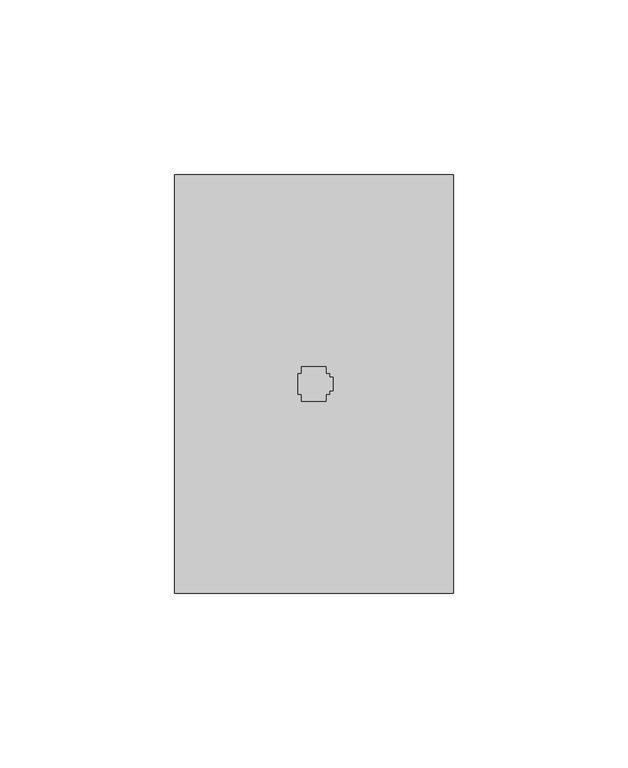
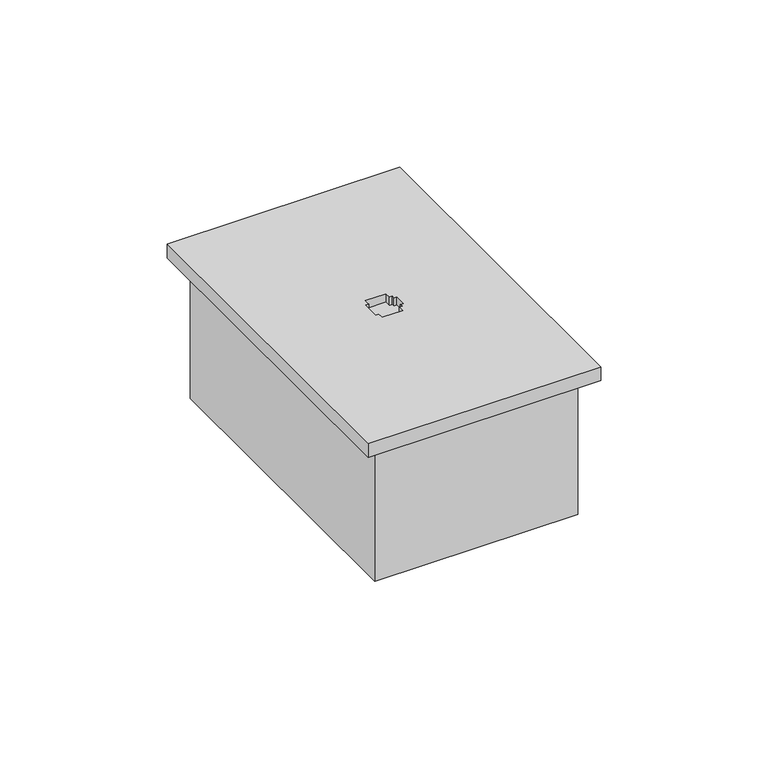
"""IFC4 building model written with IfcOpenShell, lengths in millimetres: proxy geometry, CAIXA VERTICE V7 : Telefone."""

from ifc_helpers import new_model, si_unit, origin, place, context, project, spatial, faceted_brep, source, transform, mapped, element, save


def electrical_fixtures_d1a6b59b(model_context):
    return source(origin(), model_context, "Body", "Brep", [
        faceted_brep([(33.0, 247.0, -48.0), (33.0, 353.0, -48.0), (-33.0, 353.0, -48.0), (-33.0, 247.0, -48.0), (35.0, 355.0, -50.0), (35.0, 245.0, -50.0), (-35.0, 245.0, -50.0), (-35.0, 355.0, -50.0), (-35.0, 355.0, 0.0), (35.0, 355.0, 0.0), (-35.0, 245.0, 0.0), (35.0, 245.0, 0.0), (33.0, 353.0, 0.0), (33.0, 247.0, 0.0), (-33.0, 247.0, 0.0), (-33.0, 353.0, 0.0)], [[[0, 1, 2, 3]], [[4, 5, 6, 7]], [[4, 7, 8, 9]], [[8, 7, 6, 10]], [[10, 6, 5, 11]], [[11, 5, 4, 9]], [[9, 8, 10, 11], [12, 13, 14, 15]], [[13, 12, 1, 0]], [[14, 13, 0, 3]], [[15, 14, 3, 2]], [[12, 15, 2, 1]]]),
        faceted_brep([(40.0, 360.0, 5.0), (-40.0, 360.0, 5.0), (-40.0, 240.0, 5.0), (40.0, 240.0, 5.0), (-3.5, 303.0, 5.0), (-3.5, 305.0, 5.0), (3.5, 305.0, 5.0), (3.5, 303.0, 5.0), (4.5, 303.0, 5.0), (4.5, 302.0, 5.0), (5.5, 302.0, 5.0), (5.5, 298.0, 5.0), (4.5, 298.0, 5.0), (4.5, 297.0, 5.0), (3.5, 297.0, 5.0), (3.5, 295.0, 5.0), (-3.5, 295.0, 5.0), (-3.5, 297.0, 5.0), (-4.5, 297.0, 5.0), (-4.5, 303.0, 5.0), (-40.0, 360.0, 0.0), (40.0, 360.0, 0.0), (40.0, 240.0, 0.0), (-40.0, 240.0, 0.0), (-3.5, 303.0, 2.0), (-3.5, 305.0, 2.0), (-4.5, 303.0, 2.0), (-4.5, 297.0, 2.0), (-3.5, 297.0, 2.0), (-3.5, 295.0, 2.0), (3.5, 295.0, 2.0), (3.5, 297.0, 2.0), (3.5, 305.0, 2.0), (4.5, 297.0, 2.0), (4.5, 298.0, 2.0), (5.5, 298.0, 2.0), (5.5, 302.0, 2.0), (4.5, 302.0, 2.0), (4.5, 303.0, 2.0), (3.5, 303.0, 2.0)], [[[0, 1, 2, 3], [4, 5, 6, 7, 8, 9, 10, 11, 12, 13, 14, 15, 16, 17, 18, 19]], [[20, 21, 22, 23]], [[1, 0, 21, 20]], [[2, 1, 20, 23]], [[3, 2, 23, 22]], [[0, 3, 22, 21]], [[24, 25, 5, 4]], [[26, 24, 4, 19]], [[27, 26, 19, 18]], [[28, 27, 18, 17]], [[29, 28, 17, 16]], [[30, 29, 16, 15]], [[31, 30, 15, 14]], [[32, 25, 24, 26, 27, 28, 29, 30, 31, 33, 34, 35, 36, 37, 38, 39]], [[25, 32, 6, 5]], [[33, 31, 14, 13]], [[34, 33, 13, 12]], [[35, 34, 12, 11]], [[36, 35, 11, 10]], [[37, 36, 10, 9]], [[38, 37, 9, 8]], [[39, 38, 8, 7]], [[32, 39, 7, 6]]]),
    ])


if __name__ == "__main__":
    model = new_model("IFC4")
    model_context = context("Model", 3, world=origin())
    ifc_project = project(units=[si_unit("LENGTHUNIT", "METRE", prefix="MILLI")], contexts=[model_context])
    site = spatial("IfcSite", under=ifc_project)
    building = spatial("IfcBuilding", under=site)
    placement = place(None, origin())
    electrical_fixtures_shape = electrical_fixtures_d1a6b59b(model_context)
    element("IfcBuildingElementProxy", 1, Name="CAIXA VERTICE V7 : Telefone", ObjectType="CAIXA VERTICE V7 : Telefone", at=placement, inside=building, context=model_context, shape_type="MappedRepresentation", body=[
        mapped(electrical_fixtures_shape, transform((0.0, 0.0, 0.0), x_axis=(1.0, 0.0, 0.0), y_axis=(0.0, 1.0, 0.0), z_axis=(0.0, 0.0, 1.0))),
    ])
    save(model, "model.ifc")

# Revit data of these elements
# Type "CAIXA VERTICE V7 : Telefone"
#   URL = "www.facebook.com/verticetreinamentos"
#   SEÇÃO [instance default] = ""
#   Rotação [instance default] = 0.00°
#   LARGURA DA TAMPA = 0.08 m
#   BORDA = 0.01 m
#   ALTURA DE INSTALAÇÃO [instance default] = 1.10 m
#   Distância Anotação [instance default] = 0.0015 m
#   ALTURA DA TAMPA = 0.12 m
#   Vertical [instance default] = yes
#   VER SEÇÃO [instance default] = no
#   SHADE ESQ [instance default] = no
#   SHADE DIR [instance default] = yes
#   HORIZONTAL [instance default] = no
#   ANDAR COM A LEGENDA [instance default] = 0
#   Material Tampa [instance default] = Plástico, branco opaco
#   Caixa = element 1798520
#   Anotação = element 1798519
#   Default Elevation = 0
# Element 1 (IfcBuildingElementProxy, "CAIXA VERTICE V7 : Telefone")
#   ALTURA DE INSTALAÇÃO = 0.30 m
#   SHADE DIR = no
#   Materials on its faces: "Plástico, branco opaco"
# Materials
#   "Plástico, branco opaco": class "Plástico", colour RGB 120 120 120, transparency 0, Description = "Plastic, generic, opaque white", Cost = 0
